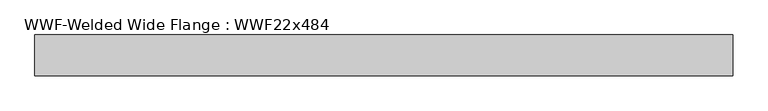
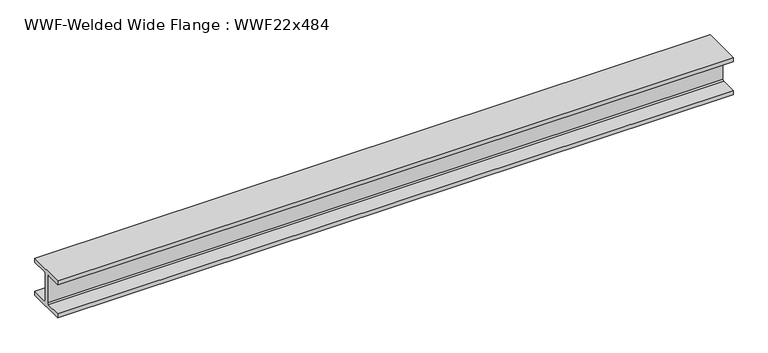
"""IFC4 building model written with IfcOpenShell, lengths in millimetres: beam geometry, WWF-Welded Wide Flange : WWF22x484."""

from ifc_helpers import new_model, si_unit, frame, origin, place, context, project, spatial, polyline, outline, extrude, source, transform, mapped, element, save


def wwf_welded_wide_flange_wwf22x484_ce9d25dd(model_context):
    return source(origin(), model_context, "Body", "SweptSolid", [
        extrude(outline(polyline([(274.955, -214.9602), (274.955, -274.955), (-274.955, -274.955), (-274.955, -214.9602), (-47.625, -214.9602), (-29.9974, -197.3326), (-29.9974, 197.3326), (-47.625, 214.9602), (-274.955, 214.9602), (-274.955, 274.955), (274.955, 274.955), (274.955, 214.9602), (47.625, 214.9602), (29.9974, 197.3326), (29.9974, -197.3326), (47.625, -214.9602), (274.955, -214.9602)])), frame((-4712.345, 0.0, 0.0), z_axis=(1.0, 0.0, 0.0), x_axis=(0.0, 1.0, 0.0)), (0.0, 0.0, 1.0), 9424.69),
    ])


if __name__ == "__main__":
    model = new_model("IFC4")
    model_context = context("Model", 3, world=origin())
    ifc_project = project(units=[si_unit("LENGTHUNIT", "METRE", prefix="MILLI")], contexts=[model_context])
    site = spatial("IfcSite", under=ifc_project)
    building = spatial("IfcBuilding", under=site)
    placement = place(None, origin())
    wwf_welded_wide_flange_wwf22x484_shape = wwf_welded_wide_flange_wwf22x484_ce9d25dd(model_context)
    element("IfcBeam", 1, ObjectType="WWF-Welded Wide Flange : WWF22x484", at=placement, inside=building, context=model_context, shape_type="MappedRepresentation", body=[
        mapped(wwf_welded_wide_flange_wwf22x484_shape, transform((0.0, 0.0, 0.0), x_axis=(1.0, 0.0, 0.0), y_axis=(0.0, 1.0, 0.0), z_axis=(0.0, 0.0, 1.0))),
    ])
    save(model, "model.ifc")

# Revit data of these elements
# Type "WWF-Welded Wide Flange : WWF22x484"
#   Assembly Code = "B10"
#   Nominal d = "12"
#   W = 484
#   Length [instance default] = 1524 mm
#   bf = 549.91 mm
#   d = 549.91 mm
#   k = 47.625 mm
#   tf = 59.995 mm
#   tw = 59.995 mm
#   A = 0.0922579 m²
#   Structural Material [instance default] = Steel ASTM A572
# Element 1 (IfcBeam, "WWF-Welded Wide Flange : WWF22x484")
#   Structural Material = Metal - Steel 43-275
#   Materials on its faces: "Metal - Steel 43-275"
# Materials
#   "Steel ASTM A572": class "Metal", colour RGB 247 247 247, transparency 0, Description = "Structural steel, high strength low alloy, ASTM - A572 - 50", Cost = 0
#   "Metal - Steel 43-275": class "Metal", colour RGB 247 247 247, transparency 0, Cost = 0
